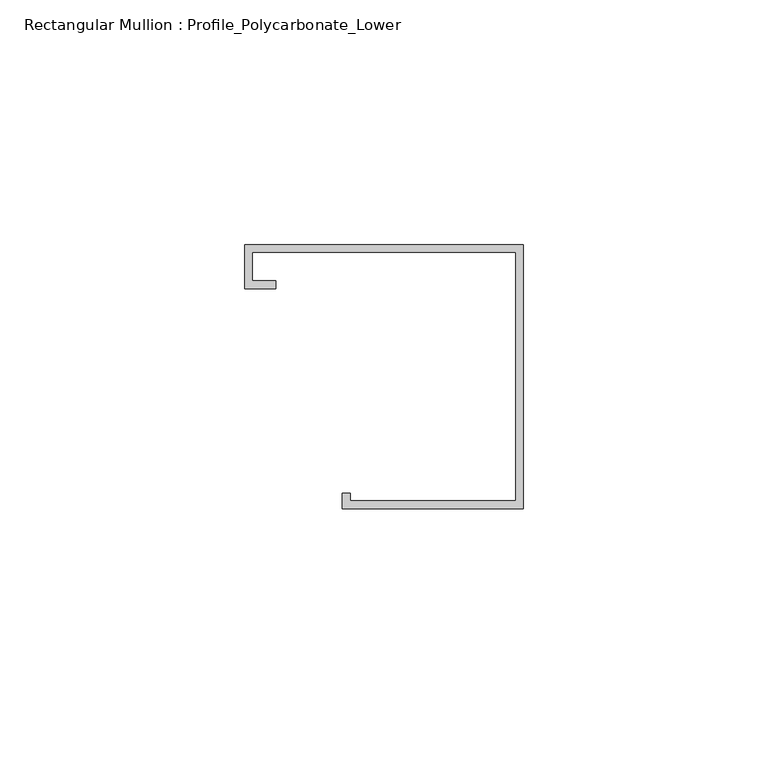
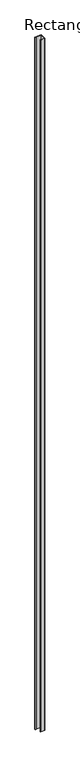
"""IFC4 building model written with IfcOpenShell, lengths in millimetres: member geometry, Rectangular Mullion : Profile_Polycarbonate_Lower."""

from ifc_helpers import new_model, si_unit, frame, origin, place, context, project, spatial, polyline, outline, extrude, source, transform, mapped, element, save


def rectangular_mullion_profile_polycarbonate_lower_7a4440f0(model_context):
    return source(origin(), model_context, "Body", "SweptSolid", [
        extrude(outline(polyline([(0.0, 28.984575), (0.0, -25.015825), (-36.9824, -25.015825), (-36.9824, -21.840825), (-35.3949, -21.840825), (-35.3949, -23.428325), (-1.5875, -23.428325), (-1.5875, 27.397075), (-55.4101, 27.397075), (-55.4101, 21.580475), (-50.6476, 21.580475), (-50.6476, 19.992975), (-56.9976, 19.992975), (-56.9976, 28.984575), (0.0, 28.984575)])), frame((0.0, 0.0, -6533.1757712), z_axis=(0.0, 0.0, 1.0), x_axis=(1.0, 0.0, 0.0)), (0.0, 0.0, 1.0), 6533.1757712),
    ])


if __name__ == "__main__":
    model = new_model("IFC4")
    model_context = context("Model", 3, world=origin())
    ifc_project = project(units=[si_unit("LENGTHUNIT", "METRE", prefix="MILLI")], contexts=[model_context])
    site = spatial("IfcSite", under=ifc_project)
    building = spatial("IfcBuilding", under=site)
    placement = place(None, origin())
    rectangular_mullion_profile_polycarbonate_lower_shape = rectangular_mullion_profile_polycarbonate_lower_7a4440f0(model_context)
    element("IfcMember", 1, ObjectType="Rectangular Mullion : Profile_Polycarbonate_Lower", at=placement, inside=building, context=model_context, shape_type="MappedRepresentation", body=[
        mapped(rectangular_mullion_profile_polycarbonate_lower_shape, transform((0.0, 0.0, 0.0), x_axis=(1.0, 0.0, 0.0), y_axis=(0.0, 1.0, 0.0), z_axis=(0.0, 0.0, 1.0))),
    ])
    save(model, "model.ifc")

# Revit data of these elements
# Type "Rectangular Mullion : Profile_Polycarbonate_Lower"
#   built-in parameter 1007322 = 0.177167 (stored number, unit not read)
#   built-in parameter 1007321 = 0 (stored number, unit not read)
#   built-in parameter 1007320 = 0.00520833 (stored number, unit not read)
